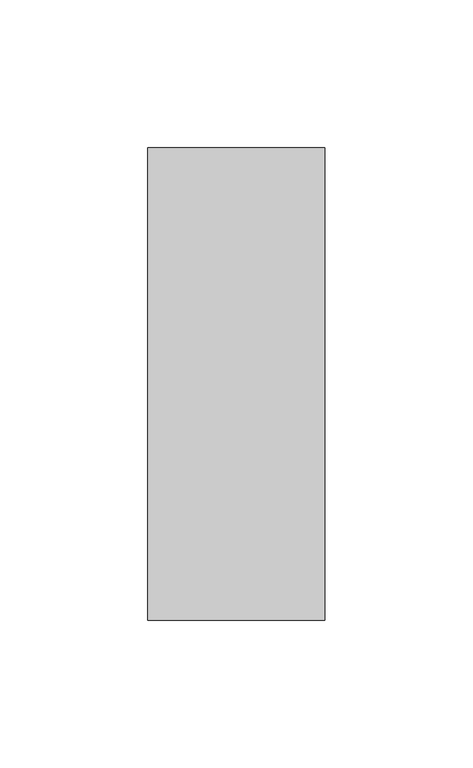
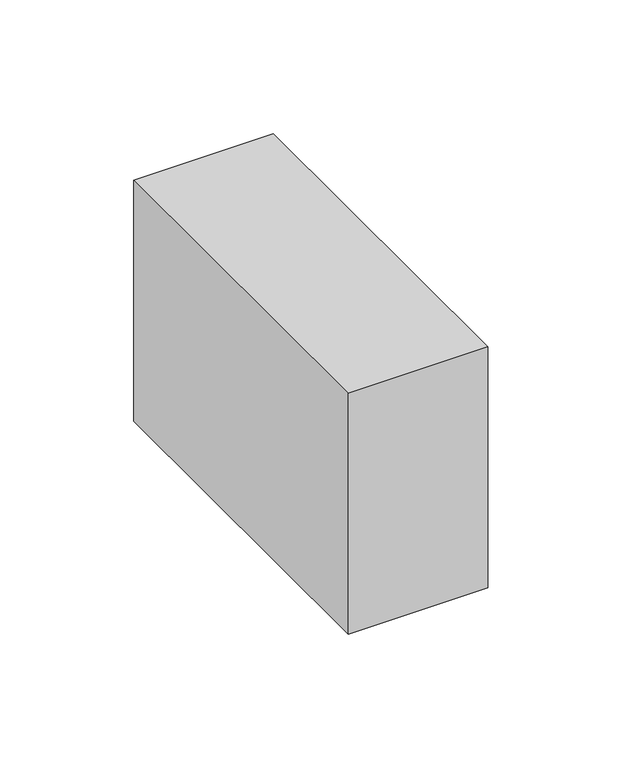
"""IFC4 building model written with IfcOpenShell, lengths in millimetres: column geometry, Madeira de lei-Coluna : Pontalete 6X16cm."""

import ifcopenshell
import ifcopenshell.guid

model = None  # the IFC model being written
_history = None  # IfcOwnerHistory: only IFC2X3 demands one
_inside = {}  # id of a spatial element -> (the spatial element, [elements in it])
_under = {}  # id of a project, library or spatial element -> (it, [spatial elements below it])
_declared = {}  # id of a project -> (the project, [libraries it declares])
_typed = {}  # id of a type object -> (the type object, [elements of that type])
_made_of = {}  # id of a material, layer set ... -> (it, [elements and type objects made of it])


def new_model(schema):
    """Start an empty IFC model of exactly this schema.

    Asked for "IFC4X3", IfcOpenShell would pick the latest addendum, in which some entities
    have other attributes; the version numbers below select the first issue.
    IFC2X3 requires an IfcOwnerHistory on every rooted entity: one is made here for all.
    """
    global model, _history
    if schema == "IFC4X3":
        model = ifcopenshell.file(schema_version=(4, 3, 0, 0))
    else:
        model = ifcopenshell.file(schema=schema)
    _inside.clear()
    _under.clear()
    _declared.clear()
    _typed.clear()
    _made_of.clear()
    _history = None
    if model.schema == "IFC2X3":
        org = make("IfcOrganization", Name="unknown")
        user = make(
            "IfcPersonAndOrganization",
            ThePerson=make("IfcPerson", FamilyName="unknown"),
            TheOrganization=org,
        )
        app = make(
            "IfcApplication",
            ApplicationDeveloper=org,
            Version="unknown",
            ApplicationFullName="unknown",
            ApplicationIdentifier="unknown",
        )
        _history = make(
            "IfcOwnerHistory",
            OwningUser=user,
            OwningApplication=app,
            ChangeAction="ADDED",
            CreationDate=0,
        )
    return model


def make(cls, **values):
    """One entity of the class cls with the attributes given. An attribute that is None is left unset."""
    return model.create_entity(
        cls, **{name: value for name, value in values.items() if value is not None}
    )


def rooted(cls, **values):
    """An entity with a GlobalId (a new one), such as an element, a storey or a relation."""
    return make(cls, GlobalId=ifcopenshell.guid.new(), OwnerHistory=_history, **values)


def si_unit(unit_type, name, prefix=None):
    """IfcSIUnit, for example si_unit("LENGTHUNIT", "METRE", prefix="MILLI")."""
    return make("IfcSIUnit", UnitType=unit_type, Prefix=prefix, Name=name)


def assignment(units):
    """IfcUnitAssignment: the units of a project."""
    return None if units is None else make("IfcUnitAssignment", Units=units)


def point(xyz):
    """IfcCartesianPoint."""
    return None if xyz is None else make("IfcCartesianPoint", Coordinates=xyz)


def direction(xyz):
    """IfcDirection."""
    return None if xyz is None else make("IfcDirection", DirectionRatios=xyz)


def frame(location, z_axis=None, x_axis=None):
    """IfcAxis2Placement3D, a coordinate frame: its origin and axes. An axis left out is left unset."""
    return make(
        "IfcAxis2Placement3D",
        Location=point(location),
        Axis=direction(z_axis),
        RefDirection=direction(x_axis),
    )


def origin():
    """The frame at (0, 0, 0) with its axes left unset."""
    return frame((0.0, 0.0, 0.0))


def place(relative_to, where):
    """IfcLocalPlacement: puts the frame where relative to a parent placement (None: the world)."""
    return make(
        "IfcLocalPlacement", PlacementRelTo=relative_to, RelativePlacement=where
    )


def context(
    kind, dimensions, precision=None, world=None, true_north=None, identifier=None
):
    """IfcGeometricRepresentationContext, for example the 3D "Model" context."""
    return make(
        "IfcGeometricRepresentationContext",
        ContextIdentifier=identifier,
        ContextType=kind,
        CoordinateSpaceDimension=dimensions,
        Precision=precision,
        WorldCoordinateSystem=world,
        TrueNorth=true_north,
    )


def project(units=None, contexts=None):
    """IfcProject with its units and contexts."""
    return rooted(
        "IfcProject",
        Name="project",
        RepresentationContexts=contexts,
        UnitsInContext=assignment(units),
    )


def spatial(cls, under=None, at=None, **own):
    """A site, building, storey or space (cls), placed at a placement, below another one or the project."""
    s = rooted(cls, ObjectPlacement=at, **own)
    if under is not None:
        _under.setdefault(under.id(), (under, []))[1].append(s)
    return s


def polyline(points):
    """IfcPolyline through the points."""
    return make("IfcPolyline", Points=[point(p) for p in points])


def outline(outer, holes=None, kind="AREA"):
    """IfcArbitraryClosedProfileDef: a profile drawn as a closed curve; with holes, ...WithVoids."""
    if holes is None:
        return make("IfcArbitraryClosedProfileDef", ProfileType=kind, OuterCurve=outer)
    return make(
        "IfcArbitraryProfileDefWithVoids",
        ProfileType=kind,
        OuterCurve=outer,
        InnerCurves=holes,
    )


def extrude(swept, where, along, depth):
    """IfcExtrudedAreaSolid: the profile swept, set in the frame where, extruded along a direction by depth."""
    return make(
        "IfcExtrudedAreaSolid",
        SweptArea=swept,
        Position=where,
        ExtrudedDirection=direction(along),
        Depth=depth,
    )


def shape(context_of_items, identifier, shape_type, items):
    """IfcShapeRepresentation: the items that make up one representation, for example the "Body"."""
    return make(
        "IfcShapeRepresentation",
        ContextOfItems=context_of_items,
        RepresentationIdentifier=identifier,
        RepresentationType=shape_type,
        Items=items,
    )


def source(mapping_origin, context_of_items, identifier, shape_type, items):
    """IfcRepresentationMap: a shape defined once, which mapped items show again and again."""
    return make(
        "IfcRepresentationMap",
        MappingOrigin=mapping_origin,
        MappedRepresentation=shape(context_of_items, identifier, shape_type, items),
    )


def transform(
    local_origin,
    x_axis=None,
    y_axis=None,
    z_axis=None,
    scale=None,
    scale2=None,
    scale3=None,
    uniform=True,
):
    """IfcCartesianTransformationOperator3D, or its non-uniform kind. x_axis, y_axis, z_axis: its Axis1, 2, 3."""
    if uniform:
        return make(
            "IfcCartesianTransformationOperator3D",
            Axis1=direction(x_axis),
            Axis2=direction(y_axis),
            LocalOrigin=point(local_origin),
            Scale=scale,
            Axis3=direction(z_axis),
        )
    return make(
        "IfcCartesianTransformationOperator3DnonUniform",
        Axis1=direction(x_axis),
        Axis2=direction(y_axis),
        LocalOrigin=point(local_origin),
        Scale=scale,
        Axis3=direction(z_axis),
        Scale2=scale2,
        Scale3=scale3,
    )


def mapped(mapping_source, mapping_target):
    """IfcMappedItem: shows the shape of a source again, moved by a transform."""
    return make(
        "IfcMappedItem", MappingSource=mapping_source, MappingTarget=mapping_target
    )


def made_of(thing, what):
    """Note that an element or type object is made of a material, layer set ...; save() writes the relation."""
    if what is not None:
        _made_of.setdefault(what.id(), (what, []))[1].append(thing)
    return thing


def element(
    cls,
    number,
    at=None,
    inside=None,
    cuts=None,
    type_object=None,
    material=None,
    context=None,
    identifier="Body",
    shape_type=None,
    held_by="IfcProductDefinitionShape",
    body=None,
    shapes=None,
    **own,
):
    """One element of the class cls, such as IfcWall. Its Tag is "e" and its number.

    at: its placement. inside: the storey or other place that contains it. cuts: it is an
    opening in that element (IfcRelVoidsElement). A single representation is given by context,
    identifier, shape_type and body (its items); several are given by shapes. held_by: the class
    of the entity that holds the representations. save() writes the other relations.
    """
    e = rooted(cls, Tag="e%d" % number, ObjectPlacement=at, **own)
    if body is not None:
        shapes = [shape(context, identifier, shape_type, body)]
    if shapes is not None:
        e.Representation = make(held_by, Representations=shapes)
    if inside is not None:
        _inside.setdefault(inside.id(), (inside, []))[1].append(e)
    if cuts is not None:
        rooted(
            "IfcRelVoidsElement", RelatingBuildingElement=cuts, RelatedOpeningElement=e
        )
    if type_object is not None:
        _typed.setdefault(type_object.id(), (type_object, []))[1].append(e)
    return made_of(e, material)


def aggregate(whole, parts):
    """IfcRelAggregates: a whole, such as a stair, and the parts it consists of."""
    return rooted("IfcRelAggregates", RelatingObject=whole, RelatedObjects=parts)


def save(model, path):
    """Write the relations noted so far, then the file.

    IfcRelAggregates (storeys below a building ...), IfcRelContainedInSpatialStructure (elements
    in a storey), IfcRelDefinesByType, IfcRelAssociatesMaterial and IfcRelDeclares: one each for
    every whole, place, type object, material and project.
    """
    for whole, parts in _under.values():
        aggregate(whole, parts)
    for where, things in _inside.values():
        rooted(
            "IfcRelContainedInSpatialStructure",
            RelatedElements=things,
            RelatingStructure=where,
        )
    for kind, things in _typed.values():
        rooted("IfcRelDefinesByType", RelatedObjects=things, RelatingType=kind)
    for what, things in _made_of.values():
        rooted("IfcRelAssociatesMaterial", RelatedObjects=things, RelatingMaterial=what)
    for by, libraries in _declared.values():
        rooted("IfcRelDeclares", RelatingContext=by, RelatedDefinitions=libraries)
    model.write(path)


def column_00c463e4(model_context):
    return source(origin(), model_context, "Body", "SweptSolid", [
        extrude(outline(polyline([(30.0, 80.0), (30.0, -80.0), (-30.0, -80.0), (-30.0, 80.0), (30.0, 80.0)])), frame((0.0, 0.0, 3110.0), z_axis=(0.0, 0.0, 1.0), x_axis=(1.0, 0.0, 0.0)), (0.0, 0.0, 1.0), 109.8),
    ])


if __name__ == "__main__":
    model = new_model("IFC4")
    model_context = context("Model", 3, world=origin())
    ifc_project = project(units=[si_unit("LENGTHUNIT", "METRE", prefix="MILLI")], contexts=[model_context])
    site = spatial("IfcSite", under=ifc_project)
    building = spatial("IfcBuilding", under=site)
    placement = place(None, origin())
    column_shape = column_00c463e4(model_context)
    element("IfcColumn", 1, ObjectType="Madeira de lei-Coluna : Pontalete 6X16cm", at=placement, inside=building, context=model_context, shape_type="MappedRepresentation", body=[
        mapped(column_shape, transform((0.0, 0.0, 0.0), x_axis=(1.0, 0.0, 0.0), y_axis=(0.0, 1.0, 0.0), z_axis=(0.0, 0.0, 1.0))),
    ])
    save(model, "model.ifc")

# Revit data of these elements
# Type "Madeira de lei-Coluna : Pontalete 6X16cm"
#   A = 0.01952 m²
#   b = 0.06 m
#   d = 0.16 m
#   Structural Material [instance default] = none
#   Assembly Code = ""
# Element 1 (IfcColumn, "Madeira de lei-Coluna : Pontalete 6X16cm")
#   Structural Material = .MADEIRAMENTO
#   Materials on its faces: ".MADEIRAMENTO"
# Materials
#   ".MADEIRAMENTO": class ".CC_MADEIRAS", colour RGB 212 179 113, transparency 0, Cost = 0
